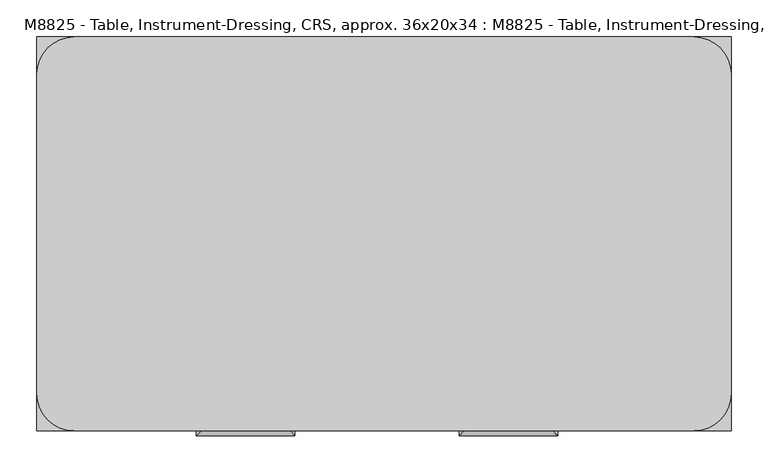
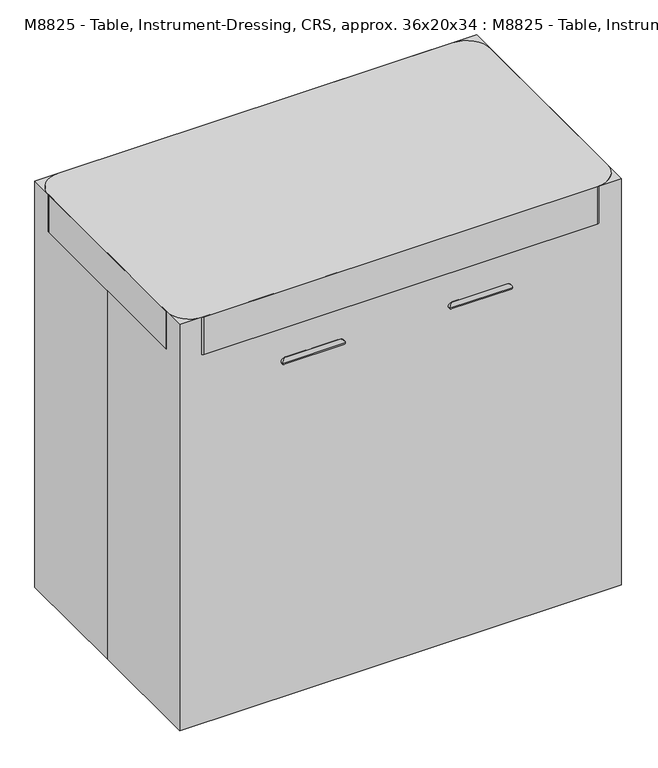
"""IFC4 building model written with IfcOpenShell, lengths in millimetres: proxy geometry, M8825 - Table, Instrument-Dressing, CRS, approx. 36x20x34 : M8825 - Table, Instrument-Dressing, CRS, approx. 36x20x34."""

import ifcopenshell
import ifcopenshell.guid

model = None  # the IFC model being written
_history = None  # IfcOwnerHistory: only IFC2X3 demands one
_inside = {}  # id of a spatial element -> (the spatial element, [elements in it])
_under = {}  # id of a project, library or spatial element -> (it, [spatial elements below it])
_declared = {}  # id of a project -> (the project, [libraries it declares])
_typed = {}  # id of a type object -> (the type object, [elements of that type])
_made_of = {}  # id of a material, layer set ... -> (it, [elements and type objects made of it])


def new_model(schema):
    """Start an empty IFC model of exactly this schema.

    Asked for "IFC4X3", IfcOpenShell would pick the latest addendum, in which some entities
    have other attributes; the version numbers below select the first issue.
    IFC2X3 requires an IfcOwnerHistory on every rooted entity: one is made here for all.
    """
    global model, _history
    if schema == "IFC4X3":
        model = ifcopenshell.file(schema_version=(4, 3, 0, 0))
    else:
        model = ifcopenshell.file(schema=schema)
    _inside.clear()
    _under.clear()
    _declared.clear()
    _typed.clear()
    _made_of.clear()
    _history = None
    if model.schema == "IFC2X3":
        org = make("IfcOrganization", Name="unknown")
        user = make(
            "IfcPersonAndOrganization",
            ThePerson=make("IfcPerson", FamilyName="unknown"),
            TheOrganization=org,
        )
        app = make(
            "IfcApplication",
            ApplicationDeveloper=org,
            Version="unknown",
            ApplicationFullName="unknown",
            ApplicationIdentifier="unknown",
        )
        _history = make(
            "IfcOwnerHistory",
            OwningUser=user,
            OwningApplication=app,
            ChangeAction="ADDED",
            CreationDate=0,
        )
    return model


def make(cls, **values):
    """One entity of the class cls with the attributes given. An attribute that is None is left unset."""
    return model.create_entity(
        cls, **{name: value for name, value in values.items() if value is not None}
    )


def rooted(cls, **values):
    """An entity with a GlobalId (a new one), such as an element, a storey or a relation."""
    return make(cls, GlobalId=ifcopenshell.guid.new(), OwnerHistory=_history, **values)


def si_unit(unit_type, name, prefix=None):
    """IfcSIUnit, for example si_unit("LENGTHUNIT", "METRE", prefix="MILLI")."""
    return make("IfcSIUnit", UnitType=unit_type, Prefix=prefix, Name=name)


def assignment(units):
    """IfcUnitAssignment: the units of a project."""
    return None if units is None else make("IfcUnitAssignment", Units=units)


def point(xyz):
    """IfcCartesianPoint."""
    return None if xyz is None else make("IfcCartesianPoint", Coordinates=xyz)


def direction(xyz):
    """IfcDirection."""
    return None if xyz is None else make("IfcDirection", DirectionRatios=xyz)


def frame(location, z_axis=None, x_axis=None):
    """IfcAxis2Placement3D, a coordinate frame: its origin and axes. An axis left out is left unset."""
    return make(
        "IfcAxis2Placement3D",
        Location=point(location),
        Axis=direction(z_axis),
        RefDirection=direction(x_axis),
    )


def frame_2d(location, x_axis=None):
    """IfcAxis2Placement2D, a coordinate frame in the plane: its origin and x axis."""
    return make(
        "IfcAxis2Placement2D", Location=point(location), RefDirection=direction(x_axis)
    )


def origin():
    """The frame at (0, 0, 0) with its axes left unset."""
    return frame((0.0, 0.0, 0.0))


def origin_with_axes():
    """The frame at (0, 0, 0) with the z axis (0, 0, 1) and the x axis (1, 0, 0) written out."""
    return frame((0.0, 0.0, 0.0), z_axis=(0.0, 0.0, 1.0), x_axis=(1.0, 0.0, 0.0))


def place(relative_to, where):
    """IfcLocalPlacement: puts the frame where relative to a parent placement (None: the world)."""
    return make(
        "IfcLocalPlacement", PlacementRelTo=relative_to, RelativePlacement=where
    )


def context(
    kind, dimensions, precision=None, world=None, true_north=None, identifier=None
):
    """IfcGeometricRepresentationContext, for example the 3D "Model" context."""
    return make(
        "IfcGeometricRepresentationContext",
        ContextIdentifier=identifier,
        ContextType=kind,
        CoordinateSpaceDimension=dimensions,
        Precision=precision,
        WorldCoordinateSystem=world,
        TrueNorth=true_north,
    )


def project(units=None, contexts=None):
    """IfcProject with its units and contexts."""
    return rooted(
        "IfcProject",
        Name="project",
        RepresentationContexts=contexts,
        UnitsInContext=assignment(units),
    )


def spatial(cls, under=None, at=None, **own):
    """A site, building, storey or space (cls), placed at a placement, below another one or the project."""
    s = rooted(cls, ObjectPlacement=at, **own)
    if under is not None:
        _under.setdefault(under.id(), (under, []))[1].append(s)
    return s


def polyline(points):
    """IfcPolyline through the points."""
    return make("IfcPolyline", Points=[point(p) for p in points])


def circle_curve(where, radius):
    """IfcCircle in the frame where."""
    return make("IfcCircle", Position=where, Radius=radius)


def ellipse_curve(where, semi_axis1, semi_axis2):
    """IfcEllipse in the frame where."""
    return make(
        "IfcEllipse", Position=where, SemiAxis1=semi_axis1, SemiAxis2=semi_axis2
    )


def trimmed(basis, trim1, trim2, sense, master):
    """IfcTrimmedCurve: the piece of a basis curve between two trims."""
    return make(
        "IfcTrimmedCurve",
        BasisCurve=basis,
        Trim1=trim1,
        Trim2=trim2,
        SenseAgreement=sense,
        MasterRepresentation=master,
    )


def segment(curve, same_sense, transition):
    """IfcCompositeCurveSegment."""
    return make(
        "IfcCompositeCurveSegment",
        Transition=transition,
        SameSense=same_sense,
        ParentCurve=curve,
    )


def composite_curve(segments, self_intersect=None):
    """IfcCompositeCurve: segments joined end to end."""
    return make("IfcCompositeCurve", Segments=segments, SelfIntersect=self_intersect)


def outline(outer, holes=None, kind="AREA"):
    """IfcArbitraryClosedProfileDef: a profile drawn as a closed curve; with holes, ...WithVoids."""
    if holes is None:
        return make("IfcArbitraryClosedProfileDef", ProfileType=kind, OuterCurve=outer)
    return make(
        "IfcArbitraryProfileDefWithVoids",
        ProfileType=kind,
        OuterCurve=outer,
        InnerCurves=holes,
    )


def extrude(swept, where, along, depth):
    """IfcExtrudedAreaSolid: the profile swept, set in the frame where, extruded along a direction by depth."""
    return make(
        "IfcExtrudedAreaSolid",
        SweptArea=swept,
        Position=where,
        ExtrudedDirection=direction(along),
        Depth=depth,
    )


def shape(context_of_items, identifier, shape_type, items):
    """IfcShapeRepresentation: the items that make up one representation, for example the "Body"."""
    return make(
        "IfcShapeRepresentation",
        ContextOfItems=context_of_items,
        RepresentationIdentifier=identifier,
        RepresentationType=shape_type,
        Items=items,
    )


def source(mapping_origin, context_of_items, identifier, shape_type, items):
    """IfcRepresentationMap: a shape defined once, which mapped items show again and again."""
    return make(
        "IfcRepresentationMap",
        MappingOrigin=mapping_origin,
        MappedRepresentation=shape(context_of_items, identifier, shape_type, items),
    )


def transform(
    local_origin,
    x_axis=None,
    y_axis=None,
    z_axis=None,
    scale=None,
    scale2=None,
    scale3=None,
    uniform=True,
):
    """IfcCartesianTransformationOperator3D, or its non-uniform kind. x_axis, y_axis, z_axis: its Axis1, 2, 3."""
    if uniform:
        return make(
            "IfcCartesianTransformationOperator3D",
            Axis1=direction(x_axis),
            Axis2=direction(y_axis),
            LocalOrigin=point(local_origin),
            Scale=scale,
            Axis3=direction(z_axis),
        )
    return make(
        "IfcCartesianTransformationOperator3DnonUniform",
        Axis1=direction(x_axis),
        Axis2=direction(y_axis),
        LocalOrigin=point(local_origin),
        Scale=scale,
        Axis3=direction(z_axis),
        Scale2=scale2,
        Scale3=scale3,
    )


def mapped(mapping_source, mapping_target):
    """IfcMappedItem: shows the shape of a source again, moved by a transform."""
    return make(
        "IfcMappedItem", MappingSource=mapping_source, MappingTarget=mapping_target
    )


def made_of(thing, what):
    """Note that an element or type object is made of a material, layer set ...; save() writes the relation."""
    if what is not None:
        _made_of.setdefault(what.id(), (what, []))[1].append(thing)
    return thing


def element(
    cls,
    number,
    at=None,
    inside=None,
    cuts=None,
    type_object=None,
    material=None,
    context=None,
    identifier="Body",
    shape_type=None,
    held_by="IfcProductDefinitionShape",
    body=None,
    shapes=None,
    **own,
):
    """One element of the class cls, such as IfcWall. Its Tag is "e" and its number.

    at: its placement. inside: the storey or other place that contains it. cuts: it is an
    opening in that element (IfcRelVoidsElement). A single representation is given by context,
    identifier, shape_type and body (its items); several are given by shapes. held_by: the class
    of the entity that holds the representations. save() writes the other relations.
    """
    e = rooted(cls, Tag="e%d" % number, ObjectPlacement=at, **own)
    if body is not None:
        shapes = [shape(context, identifier, shape_type, body)]
    if shapes is not None:
        e.Representation = make(held_by, Representations=shapes)
    if inside is not None:
        _inside.setdefault(inside.id(), (inside, []))[1].append(e)
    if cuts is not None:
        rooted(
            "IfcRelVoidsElement", RelatingBuildingElement=cuts, RelatedOpeningElement=e
        )
    if type_object is not None:
        _typed.setdefault(type_object.id(), (type_object, []))[1].append(e)
    return made_of(e, material)


def aggregate(whole, parts):
    """IfcRelAggregates: a whole, such as a stair, and the parts it consists of."""
    return rooted("IfcRelAggregates", RelatingObject=whole, RelatedObjects=parts)


def save(model, path):
    """Write the relations noted so far, then the file.

    IfcRelAggregates (storeys below a building ...), IfcRelContainedInSpatialStructure (elements
    in a storey), IfcRelDefinesByType, IfcRelAssociatesMaterial and IfcRelDeclares: one each for
    every whole, place, type object, material and project.
    """
    for whole, parts in _under.values():
        aggregate(whole, parts)
    for where, things in _inside.values():
        rooted(
            "IfcRelContainedInSpatialStructure",
            RelatedElements=things,
            RelatingStructure=where,
        )
    for kind, things in _typed.values():
        rooted("IfcRelDefinesByType", RelatedObjects=things, RelatingType=kind)
    for what, things in _made_of.values():
        rooted("IfcRelAssociatesMaterial", RelatedObjects=things, RelatingMaterial=what)
    for by, libraries in _declared.values():
        rooted("IfcRelDeclares", RelatingContext=by, RelatedDefinitions=libraries)
    model.write(path)


def plane_surface(at):
    """IfcPlane: the flat surface through the origin of the frame at, square to its z axis."""
    return make("IfcPlane", Position=at)


def cylinder_surface(at, radius):
    """IfcCylindricalSurface: all points at the distance radius from the z axis of the frame at."""
    return make("IfcCylindricalSurface", Position=at, Radius=radius)


def advanced_brep(points, edges, surfaces, faces):
    """IfcAdvancedBrep: a solid bounded by faces that lie on surfaces and meet in shared edges.

    An edge is (start, end): straight between two places in points (the first is 0);
    or (start, end, curve); or (start, end, curve, False) where it runs against its curve.
    A face is (place in surfaces, loops), or (place, loops, False) where it looks against
    its surface's normal. A loop lists edges by number (the first is 1), with a minus sign
    where the edge is run from its end to its start. The first loop is the outer one.
    """
    corners = [point(p) for p in points]
    vertices = [make("IfcVertexPoint", VertexGeometry=c) for c in corners]
    made = []
    for start, end, *more in edges:
        made.append(
            make(
                "IfcEdgeCurve",
                EdgeStart=vertices[start],
                EdgeEnd=vertices[end],
                EdgeGeometry=more[0] if more else make("IfcPolyline", Points=[corners[start], corners[end]]),
                SameSense=more[1] if len(more) > 1 else True,
            )
        )
    hull = []
    for where, loops, *sense in faces:
        bounds = []
        for j, loop in enumerate(loops):
            ring = [make("IfcOrientedEdge", EdgeElement=made[abs(k) - 1], Orientation=k > 0) for k in loop]
            bounds.append(
                make(
                    "IfcFaceOuterBound" if j == 0 else "IfcFaceBound",
                    Bound=make("IfcEdgeLoop", EdgeList=ring),
                    Orientation=True,
                )
            )
        hull.append(make("IfcAdvancedFace", Bounds=bounds, FaceSurface=surfaces[where], SameSense=sense[0] if sense else True))
    return make("IfcAdvancedBrep", Outer=make("IfcClosedShell", CfsFaces=hull))


def m8825_table_instrument_dressing_crs_approx_36x20x34_m8825_21174694(model_context):
    return source(origin(), model_context, "Body", "SolidModel", [
        extrude(outline(polyline([(-349.25, 174.4117179), (-349.25, 212.5117179), (349.25, 212.5117179), (349.25, 174.4117179), (400.05, 174.4117179), (400.05, -171.4283546), (349.25, -171.4283546), (349.25, -209.5283546), (-349.25, -209.5283546), (-349.25, -171.4283546), (-400.05, -171.4283546), (-400.05, 174.4117179), (-349.25, 174.4117179)])), frame((0.0, 0.0, 292.1), z_axis=(0.0, 0.0, 1.0), x_axis=(1.0, 0.0, 0.0)), (0.0, 0.0, 1.0), 38.1),
        advanced_brep(
        [(101.6, -228.5783546, 755.65), (114.3, -228.5783546, 755.65), (101.6, -273.05, 755.65), (114.3, -260.35, 755.65), (234.95, -273.05, 755.65), (222.25, -260.35, 755.65), (234.95, -228.5783546, 755.65), (222.25, -228.5783546, 755.65)],
        [
            (0, 1, circle_curve(frame((107.95, -228.5783546, 755.65), z_axis=(0.0, 1.0, 0.0), x_axis=(1.0, 0.0, 0.0)), 6.35)),
            (1, 0, circle_curve(frame((107.95, -228.5783546, 755.65), z_axis=(0.0, 1.0, 0.0), x_axis=(1.0, 0.0, 0.0)), 6.35)),
            (0, 2),
            (2, 3, ellipse_curve(frame((107.95, -266.7, 755.65), z_axis=(-0.7071067811865457, 0.7071067811865492, 0.0), x_axis=(0.7071067811865491, 0.7071067811865458, 0.0)), 8.9802561, 6.35)),
            (3, 1),
            (3, 2, ellipse_curve(frame((107.95, -266.7, 755.65), z_axis=(-0.7071067811865457, 0.7071067811865492, 0.0), x_axis=(0.7071067811865491, 0.7071067811865458, 0.0)), 8.9802561, 6.35)),
            (2, 4),
            (4, 5, ellipse_curve(frame((228.6, -266.7, 755.65), z_axis=(-0.7071067811865492, -0.7071067811865457, 0.0), x_axis=(-0.7071067811865458, 0.7071067811865492, 0.0)), 8.9802561, 6.35)),
            (5, 3),
            (5, 4, ellipse_curve(frame((228.6, -266.7, 755.65), z_axis=(-0.7071067811865492, -0.7071067811865457, 0.0), x_axis=(-0.7071067811865458, 0.7071067811865492, 0.0)), 8.9802561, 6.35)),
            (6, 7, circle_curve(frame((228.6, -228.5783546, 755.65), z_axis=(0.0, 1.0, 0.0), x_axis=(-1.0, 0.0, 0.0)), 6.35)),
            (7, 6, circle_curve(frame((228.6, -228.5783546, 755.65), z_axis=(0.0, 1.0, 0.0), x_axis=(-1.0, 0.0, 0.0)), 6.35)),
            (4, 6),
            (7, 5),
        ],
        [
            plane_surface(frame((107.95, -228.5783546, 755.65), z_axis=(0.0, 1.0, 0.0), x_axis=(0.0, 0.0, 1.0))),
            cylinder_surface(frame((107.95, -228.5783546, 755.65), z_axis=(0.0, 1.0, 0.0), x_axis=(1.0, 0.0, 0.0)), 6.35),
            cylinder_surface(frame((107.95, -266.7, 755.65), z_axis=(-1.0, 0.0, 0.0), x_axis=(0.0, 1.0, 0.0)), 6.35),
            plane_surface(frame((228.6, -228.5783546, 755.65), z_axis=(0.0, 1.0, 0.0), x_axis=(0.0, 0.0, 1.0))),
            cylinder_surface(frame((228.6, -266.7, 755.65), z_axis=(0.0, -1.0, 0.0), x_axis=(-1.0, 0.0, 0.0)), 6.35),
        ],
        [
            (0, [[1, 2]]),
            (1, [[-1, 3, 4, 5]]),
            (1, [[-2, -5, 6, -3]]),
            (2, [[-4, 7, 8, 9]]),
            (2, [[-6, -9, 10, -7]]),
            (3, [[11, 12]]),
            (4, [[-8, 13, -12, 14]]),
            (4, [[-10, -14, -11, -13]]),
        ],
    ),
        extrude(outline(polyline([(328.7951144, -228.5783546), (23.9951144, -228.5783546), (23.9951144, -209.5283546), (328.7951144, -209.5283546), (328.7951144, -228.5783546)])), frame((0.0, 0.0, 714.264534), z_axis=(0.0, 0.0, 1.0), x_axis=(1.0, 0.0, 0.0)), (0.0, 0.0, 1.0), 88.9),
        advanced_brep(
        [(-254.0, -228.5783546, 755.65), (-241.3, -228.5783546, 755.65), (-254.0, -273.05, 755.65), (-241.3, -260.35, 755.65), (-120.65, -273.05, 755.65), (-133.35, -260.35, 755.65), (-120.65, -228.5783546, 755.65), (-133.35, -228.5783546, 755.65)],
        [
            (0, 1, circle_curve(frame((-247.65, -228.5783546, 755.65), z_axis=(0.0, 1.0, 0.0), x_axis=(1.0, 0.0, 0.0)), 6.35)),
            (1, 0, circle_curve(frame((-247.65, -228.5783546, 755.65), z_axis=(0.0, 1.0, 0.0), x_axis=(1.0, 0.0, 0.0)), 6.35)),
            (0, 2),
            (2, 3, ellipse_curve(frame((-247.65, -266.7, 755.65), z_axis=(-0.7071067811865457, 0.7071067811865492, 0.0), x_axis=(0.7071067811865491, 0.7071067811865458, 0.0)), 8.9802561, 6.35)),
            (3, 1),
            (3, 2, ellipse_curve(frame((-247.65, -266.7, 755.65), z_axis=(-0.7071067811865457, 0.7071067811865492, 0.0), x_axis=(0.7071067811865491, 0.7071067811865458, 0.0)), 8.9802561, 6.35)),
            (2, 4),
            (4, 5, ellipse_curve(frame((-127.0, -266.7, 755.65), z_axis=(-0.7071067811865492, -0.7071067811865457, 0.0), x_axis=(-0.7071067811865458, 0.7071067811865492, 0.0)), 8.9802561, 6.35)),
            (5, 3),
            (5, 4, ellipse_curve(frame((-127.0, -266.7, 755.65), z_axis=(-0.7071067811865492, -0.7071067811865457, 0.0), x_axis=(-0.7071067811865458, 0.7071067811865492, 0.0)), 8.9802561, 6.35)),
            (6, 7, circle_curve(frame((-127.0, -228.5783546, 755.65), z_axis=(0.0, 1.0, 0.0), x_axis=(-1.0, 0.0, 0.0)), 6.35)),
            (7, 6, circle_curve(frame((-127.0, -228.5783546, 755.65), z_axis=(0.0, 1.0, 0.0), x_axis=(-1.0, 0.0, 0.0)), 6.35)),
            (4, 6),
            (7, 5),
        ],
        [
            plane_surface(frame((-247.65, -228.5783546, 755.65), z_axis=(0.0, 1.0, 0.0), x_axis=(0.0, 0.0, 1.0))),
            cylinder_surface(frame((-247.65, -228.5783546, 755.65), z_axis=(0.0, 1.0, 0.0), x_axis=(1.0, 0.0, 0.0)), 6.35),
            cylinder_surface(frame((-247.65, -266.7, 755.65), z_axis=(-1.0, 0.0, 0.0), x_axis=(0.0, 1.0, 0.0)), 6.35),
            plane_surface(frame((-127.0, -228.5783546, 755.65), z_axis=(0.0, 1.0, 0.0), x_axis=(0.0, 0.0, 1.0))),
            cylinder_surface(frame((-127.0, -266.7, 755.65), z_axis=(0.0, -1.0, 0.0), x_axis=(-1.0, 0.0, 0.0)), 6.35),
        ],
        [
            (0, [[1, 2]]),
            (1, [[-1, 3, 4, 5]]),
            (1, [[-2, -5, 6, -3]]),
            (2, [[-4, 7, 8, 9]]),
            (2, [[-6, -9, 10, -7]]),
            (3, [[11, 12]]),
            (4, [[-8, 13, -12, 14]]),
            (4, [[-10, -14, -11, -13]]),
        ],
    ),
        extrude(outline(polyline([(-26.8048856, -228.5783546), (-331.6048856, -228.5783546), (-331.6048856, -209.5283546), (-26.8048856, -209.5283546), (-26.8048856, -228.5783546)])), frame((0.0, 0.0, 714.264534), z_axis=(0.0, 0.0, 1.0), x_axis=(1.0, 0.0, 0.0)), (0.0, 0.0, 1.0), 88.9),
        extrude(outline(polyline([(349.25, 193.4617179), (-349.25, 193.4617179), (-349.25, 212.5117179), (349.25, 212.5117179), (349.25, 193.4617179)])), frame((0.0, 0.0, 690.1016667), z_axis=(0.0, 0.0, 1.0), x_axis=(1.0, 0.0, 0.0)), (0.0, 0.0, 1.0), 139.7),
        extrude(outline(polyline([(349.25, -209.5283546), (-349.25, -209.5283546), (-349.25, -190.4783546), (349.25, -190.4783546), (349.25, -209.5283546)])), frame((0.0, 0.0, 690.1016667), z_axis=(0.0, 0.0, 1.0), x_axis=(1.0, 0.0, 0.0)), (0.0, 0.0, 1.0), 139.7),
        extrude(outline(polyline([(381.0, -171.4283546), (381.0, 174.4117179), (400.05, 174.4117179), (400.05, -171.4283546), (381.0, -171.4283546)])), frame((0.0, 0.0, 690.1016667), z_axis=(0.0, 0.0, 1.0), x_axis=(1.0, 0.0, 0.0)), (0.0, 0.0, 1.0), 139.7),
        extrude(outline(polyline([(-381.0, 174.4117179), (-381.0, -171.4283546), (-400.05, -171.4283546), (-400.05, 174.4117179), (-381.0, 174.4117179)])), frame((0.0, 0.0, 690.1016667), z_axis=(0.0, 0.0, 1.0), x_axis=(1.0, 0.0, 0.0)), (0.0, 0.0, 1.0), 139.7),
        extrude(outline(polyline([(349.25, -209.5283546), (349.25, -171.4283546), (400.05, -171.4283546), (400.05, -209.5283546), (349.25, -209.5283546)])), frame((0.0, 0.0, 127.0), z_axis=(0.0, 0.0, 1.0), x_axis=(1.0, 0.0, 0.0)), (0.0, 0.0, 1.0), 702.8016667),
        extrude(outline(polyline([(349.25, 212.5117179), (400.05, 212.5117179), (400.05, 174.4117179), (349.25, 174.4117179), (349.25, 212.5117179)])), frame((0.0, 0.0, 127.0), z_axis=(0.0, 0.0, 1.0), x_axis=(1.0, 0.0, 0.0)), (0.0, 0.0, 1.0), 702.8016667),
        extrude(outline(polyline([(-349.25, -209.5283546), (-400.05, -209.5283546), (-400.05, -171.4283546), (-349.25, -171.4283546), (-349.25, -209.5283546)])), frame((0.0, 0.0, 127.0), z_axis=(0.0, 0.0, 1.0), x_axis=(1.0, 0.0, 0.0)), (0.0, 0.0, 1.0), 702.8016667),
        extrude(outline(polyline([(-349.25, 212.5117179), (-349.25, 174.4117179), (-400.05, 174.4117179), (-400.05, 212.5117179), (-349.25, 212.5117179)])), frame((0.0, 0.0, 127.0), z_axis=(0.0, 0.0, 1.0), x_axis=(1.0, 0.0, 0.0)), (0.0, 0.0, 1.0), 702.8016667),
        extrude(outline(composite_curve([segment(trimmed(circle_curve(frame_2d((-366.1833333, 193.6533546)), 16.9333333), [point((-366.1833333, 210.5866879))], [point((-366.1833333, 176.7200213))], False, "CARTESIAN"), True, "CONTINUOUS"), segment(trimmed(circle_curve(frame_2d((-366.1833333, 193.6533546)), 16.9333333), [point((-366.1833333, 176.7200213))], [point((-366.1833333, 210.5866879))], False, "CARTESIAN"), True, "CONTINUOUS")], self_intersect=False)), frame((0.0, 0.0, 84.8149176), z_axis=(0.0, 0.0, 1.0), x_axis=(1.0, 0.0, 0.0)), (0.0, 0.0, 1.0), 42.1850824),
        extrude(outline(composite_curve([segment(trimmed(circle_curve(frame_2d((-366.1833333, -190.4783546)), 16.9333333), [point((-366.1833333, -207.4116879))], [point((-366.1833333, -173.5450213))], False, "CARTESIAN"), True, "CONTINUOUS"), segment(trimmed(circle_curve(frame_2d((-366.1833333, -190.4783546)), 16.9333333), [point((-366.1833333, -173.5450213))], [point((-366.1833333, -207.4116879))], False, "CARTESIAN"), True, "CONTINUOUS")], self_intersect=False)), frame((0.0, 0.0, 84.8149176), z_axis=(0.0, 0.0, 1.0), x_axis=(1.0, 0.0, 0.0)), (0.0, 0.0, 1.0), 42.1850824),
        extrude(outline(composite_curve([segment(trimmed(circle_curve(frame_2d((50.8, -349.25)), 50.8), [point((50.8, -400.05))], [point((50.8, -298.45))], False, "CARTESIAN"), True, "CONTINUOUS"), segment(trimmed(circle_curve(frame_2d((50.8, -349.25)), 50.8), [point((50.8, -298.45))], [point((50.8, -400.05))], False, "CARTESIAN"), True, "CONTINUOUS")], self_intersect=False)), frame((0.0, -171.45, 0.0), z_axis=(0.0, 1.0, 0.0), x_axis=(0.0, 0.0, 1.0)), (0.0, 0.0, 1.0), 19.05),
        extrude(outline(composite_curve([segment(trimmed(circle_curve(frame_2d((50.8, -349.25)), 50.8), [point((50.8, -400.05))], [point((50.8, -298.45))], False, "CARTESIAN"), True, "CONTINUOUS"), segment(trimmed(circle_curve(frame_2d((50.8, -349.25)), 50.8), [point((50.8, -298.45))], [point((50.8, -400.05))], False, "CARTESIAN"), True, "CONTINUOUS")], self_intersect=False)), frame((0.0, -228.6, 0.0), z_axis=(0.0, 1.0, 0.0), x_axis=(0.0, 0.0, 1.0)), (0.0, 0.0, 1.0), 19.05),
        extrude(outline(composite_curve([segment(trimmed(circle_curve(frame_2d((50.8, -349.25)), 33.8666667), [point((50.8, -315.3833333))], [point((50.8, -383.1166667))], False, "CARTESIAN"), True, "CONTINUOUS"), segment(trimmed(circle_curve(frame_2d((50.8, -349.25)), 33.8666667), [point((50.8, -383.1166667))], [point((50.8, -315.3833333))], False, "CARTESIAN"), True, "CONTINUOUS")], self_intersect=False)), frame((0.0, -209.55, 0.0), z_axis=(0.0, 1.0, 0.0), x_axis=(0.0, 0.0, 1.0)), (0.0, 0.0, 1.0), 38.1),
        extrude(outline(composite_curve([segment(trimmed(circle_curve(frame_2d((50.8, -349.25)), 50.8), [point((50.8, -400.05))], [point((50.8, -298.45))], False, "CARTESIAN"), True, "CONTINUOUS"), segment(trimmed(circle_curve(frame_2d((50.8, -349.25)), 50.8), [point((50.8, -298.45))], [point((50.8, -400.05))], False, "CARTESIAN"), True, "CONTINUOUS")], self_intersect=False)), frame((0.0, 155.3617179, 0.0), z_axis=(0.0, 1.0, 0.0), x_axis=(0.0, 0.0, 1.0)), (0.0, 0.0, 1.0), 19.05),
        extrude(outline(composite_curve([segment(trimmed(circle_curve(frame_2d((50.8, -349.25)), 50.8), [point((50.8, -400.05))], [point((50.8, -298.45))], False, "CARTESIAN"), True, "CONTINUOUS"), segment(trimmed(circle_curve(frame_2d((50.8, -349.25)), 50.8), [point((50.8, -298.45))], [point((50.8, -400.05))], False, "CARTESIAN"), True, "CONTINUOUS")], self_intersect=False)), frame((0.0, 212.5117179, 0.0), z_axis=(0.0, 1.0, 0.0), x_axis=(0.0, 0.0, 1.0)), (0.0, 0.0, 1.0), 19.05),
        extrude(outline(composite_curve([segment(trimmed(circle_curve(frame_2d((50.8, -349.25)), 33.8666667), [point((50.8, -315.3833333))], [point((50.8, -383.1166667))], False, "CARTESIAN"), True, "CONTINUOUS"), segment(trimmed(circle_curve(frame_2d((50.8, -349.25)), 33.8666667), [point((50.8, -383.1166667))], [point((50.8, -315.3833333))], False, "CARTESIAN"), True, "CONTINUOUS")], self_intersect=False)), frame((0.0, 174.4117179, 0.0), z_axis=(0.0, 1.0, 0.0), x_axis=(0.0, 0.0, 1.0)), (0.0, 0.0, 1.0), 38.1),
        extrude(outline(composite_curve([segment(trimmed(circle_curve(frame_2d((366.1833333, 193.6533546)), 16.9333333), [point((366.1833333, 210.5866879))], [point((366.1833333, 176.7200213))], False, "CARTESIAN"), True, "CONTINUOUS"), segment(trimmed(circle_curve(frame_2d((366.1833333, 193.6533546)), 16.9333333), [point((366.1833333, 176.7200213))], [point((366.1833333, 210.5866879))], False, "CARTESIAN"), True, "CONTINUOUS")], self_intersect=False)), frame((0.0, 0.0, 84.8149176), z_axis=(0.0, 0.0, 1.0), x_axis=(1.0, 0.0, 0.0)), (0.0, 0.0, 1.0), 42.1850824),
        extrude(outline(composite_curve([segment(trimmed(circle_curve(frame_2d((366.1833333, -190.4783546)), 16.9333333), [point((366.1833333, -207.4116879))], [point((366.1833333, -173.5450213))], False, "CARTESIAN"), True, "CONTINUOUS"), segment(trimmed(circle_curve(frame_2d((366.1833333, -190.4783546)), 16.9333333), [point((366.1833333, -173.5450213))], [point((366.1833333, -207.4116879))], False, "CARTESIAN"), True, "CONTINUOUS")], self_intersect=False)), frame((0.0, 0.0, 84.8149176), z_axis=(0.0, 0.0, 1.0), x_axis=(1.0, 0.0, 0.0)), (0.0, 0.0, 1.0), 42.1850824),
        extrude(outline(composite_curve([segment(trimmed(circle_curve(frame_2d((50.8, 349.25)), 50.8), [point((50.8, 400.05))], [point((50.8, 298.45))], False, "CARTESIAN"), True, "CONTINUOUS"), segment(trimmed(circle_curve(frame_2d((50.8, 349.25)), 50.8), [point((50.8, 298.45))], [point((50.8, 400.05))], False, "CARTESIAN"), True, "CONTINUOUS")], self_intersect=False)), frame((0.0, -171.45, 0.0), z_axis=(0.0, 1.0, 0.0), x_axis=(0.0, 0.0, 1.0)), (0.0, 0.0, 1.0), 19.05),
        extrude(outline(composite_curve([segment(trimmed(circle_curve(frame_2d((50.8, 349.25)), 50.8), [point((50.8, 400.05))], [point((50.8, 298.45))], False, "CARTESIAN"), True, "CONTINUOUS"), segment(trimmed(circle_curve(frame_2d((50.8, 349.25)), 50.8), [point((50.8, 298.45))], [point((50.8, 400.05))], False, "CARTESIAN"), True, "CONTINUOUS")], self_intersect=False)), frame((0.0, -228.6, 0.0), z_axis=(0.0, 1.0, 0.0), x_axis=(0.0, 0.0, 1.0)), (0.0, 0.0, 1.0), 19.05),
        extrude(outline(composite_curve([segment(trimmed(circle_curve(frame_2d((50.8, 349.25)), 33.8666667), [point((50.8, 315.3833333))], [point((50.8, 383.1166667))], False, "CARTESIAN"), True, "CONTINUOUS"), segment(trimmed(circle_curve(frame_2d((50.8, 349.25)), 33.8666667), [point((50.8, 383.1166667))], [point((50.8, 315.3833333))], False, "CARTESIAN"), True, "CONTINUOUS")], self_intersect=False)), frame((0.0, -209.55, 0.0), z_axis=(0.0, 1.0, 0.0), x_axis=(0.0, 0.0, 1.0)), (0.0, 0.0, 1.0), 38.1),
        extrude(outline(composite_curve([segment(trimmed(circle_curve(frame_2d((50.8, 349.25)), 50.8), [point((50.8, 400.05))], [point((50.8, 298.45))], False, "CARTESIAN"), True, "CONTINUOUS"), segment(trimmed(circle_curve(frame_2d((50.8, 349.25)), 50.8), [point((50.8, 298.45))], [point((50.8, 400.05))], False, "CARTESIAN"), True, "CONTINUOUS")], self_intersect=False)), frame((0.0, 155.3617179, 0.0), z_axis=(0.0, 1.0, 0.0), x_axis=(0.0, 0.0, 1.0)), (0.0, 0.0, 1.0), 19.05),
        extrude(outline(composite_curve([segment(trimmed(circle_curve(frame_2d((50.8, 349.25)), 50.8), [point((50.8, 400.05))], [point((50.8, 298.45))], False, "CARTESIAN"), True, "CONTINUOUS"), segment(trimmed(circle_curve(frame_2d((50.8, 349.25)), 50.8), [point((50.8, 298.45))], [point((50.8, 400.05))], False, "CARTESIAN"), True, "CONTINUOUS")], self_intersect=False)), frame((0.0, 212.5117179, 0.0), z_axis=(0.0, 1.0, 0.0), x_axis=(0.0, 0.0, 1.0)), (0.0, 0.0, 1.0), 19.05),
        extrude(outline(composite_curve([segment(trimmed(circle_curve(frame_2d((50.8, 349.25)), 33.8666667), [point((50.8, 315.3833333))], [point((50.8, 383.1166667))], False, "CARTESIAN"), True, "CONTINUOUS"), segment(trimmed(circle_curve(frame_2d((50.8, 349.25)), 33.8666667), [point((50.8, 383.1166667))], [point((50.8, 315.3833333))], False, "CARTESIAN"), True, "CONTINUOUS")], self_intersect=False)), frame((0.0, 174.4117179, 0.0), z_axis=(0.0, 1.0, 0.0), x_axis=(0.0, 0.0, 1.0)), (0.0, 0.0, 1.0), 38.1),
        extrude(outline(composite_curve([segment(trimmed(circle_curve(frame_2d((419.1, 215.9)), 50.8), [point((419.1, 266.7))], [point((469.9, 215.9))], False, "CARTESIAN"), True, "CONTINUOUS"), segment(polyline([(469.9, 215.9), (469.9, -215.9)]), True, "CONTINUOUS"), segment(trimmed(circle_curve(frame_2d((419.1, -215.9)), 50.8), [point((469.9, -215.9))], [point((419.1, -266.7))], False, "CARTESIAN"), True, "CONTINUOUS"), segment(polyline([(419.1, -266.7), (-419.1, -266.7)]), True, "CONTINUOUS"), segment(trimmed(circle_curve(frame_2d((-419.1, -215.9)), 50.8), [point((-419.1, -266.7))], [point((-469.9, -215.9))], False, "CARTESIAN"), True, "CONTINUOUS"), segment(polyline([(-469.9, -215.9), (-469.9, 215.9)]), True, "CONTINUOUS"), segment(trimmed(circle_curve(frame_2d((-419.1, 215.9)), 50.8), [point((-469.9, 215.9))], [point((-419.1, 266.7))], False, "CARTESIAN"), True, "CONTINUOUS"), segment(polyline([(-419.1, 266.7), (419.1, 266.7)]), True, "CONTINUOUS")], self_intersect=False)), frame((0.0, 0.0, 829.8016667), z_axis=(0.0, 0.0, 1.0), x_axis=(1.0, 0.0, 0.0)), (0.0, 0.0, 1.0), 84.5983333),
        extrude(outline(polyline([(-469.9, 266.7), (469.9, 266.7), (469.9, -266.7), (-469.9, -266.7), (-469.9, 0.0), (-469.9, 266.7)])), origin_with_axes(), (0.0, 0.0, 1.0), 914.4),
    ])


if __name__ == "__main__":
    model = new_model("IFC4")
    model_context = context("Model", 3, world=origin())
    ifc_project = project(units=[si_unit("LENGTHUNIT", "METRE", prefix="MILLI")], contexts=[model_context])
    site = spatial("IfcSite", under=ifc_project)
    building = spatial("IfcBuilding", under=site)
    placement = place(None, origin())
    m8825_table_instrument_dressing_crs_approx_36x20x34_m8825_shape = m8825_table_instrument_dressing_crs_approx_36x20x34_m8825_21174694(model_context)
    element("IfcBuildingElementProxy", 1, Name="M8825 - Table, Instrument-Dressing, CRS, approx. 36x20x34 : M8825 - Table, Instrument-Dressing, CRS, approx. 36x20x34", ObjectType="M8825 - Table, Instrument-Dressing, CRS, approx. 36x20x34 : M8825 - Table, Instrument-Dressing, CRS, approx. 36x20x34", at=placement, inside=building, context=model_context, shape_type="MappedRepresentation", body=[
        mapped(m8825_table_instrument_dressing_crs_approx_36x20x34_m8825_shape, transform((0.0, 0.0, 0.0), x_axis=(1.0, 0.0, 0.0), y_axis=(0.0, 1.0, 0.0), z_axis=(0.0, 0.0, 1.0))),
    ])
    save(model, "model.ifc")

# Revit data of these elements
# Project information
#   Room Abbreviation = "XDCY1"
#   Room Description = "Xray, Cystology (XDCY1)"
#   Sheets - Total = "6"
#   Project Issue Date = "Issue Date"
#   Project Status = "Project Status"
#   Client Name = "Owner"
#   Project Address = "Enter address here"
#   Project Name = "Project Name"
#   Project Number = "Project Number"
#   Publication Date = "1-Feb-16"
# Type "M8825 - Table, Instrument-Dressing, CRS, approx. 36x20x34 : M8825 - Table, Instrument-Dressing, CRS, approx. 36x20x34"
#   Watts2 = "0"
#   Watts1 = "0"
#   Unit_Issue = "EA"
#   UTIL_6_Misc = "-"
#   UTIL_5_NonMedGas = "-"
#   UTIL_4_MiscGas = "-"
#   UTIL_3_MedGas = "-"
#   UTIL_2_Elec = "-"
#   UTIL_1_WaterDrain = "-"
#   Nomenclature = "Table, Instrument/Dressing, CRS, approx. 36x20x34"
#   NSN = "6530"
#   Location [instance default] = ""
#   JSN = "M8825"
#   Fund_Source_VA = "-"
#   Fund_Source_Navy = "-"
#   Fund_Source_Army = "-"
#   Fund_Source_AF = "-"
#   ELEC_Volts2 = "0"
#   ELEC_Volts1 = "0"
#   ELEC_Phase2 = "0"
#   ELEC_Phase1 = "0"
#   ELEC_HertzSwitch = "0"
#   ELEC_HertzDependent = "0"
#   ELEC_Hertz = "0"
#   ELEC_Amps2 = "0"
#   ELEC_Amps1 = "0"
#   DetailDescription = "Instrument and dressing table. Made of corrosion resistant stainless steel with a sound deadened top. Includes guard rail, shelf and two side-by-side drawers. The table is mounted on swivel, ball-bearing casters."
#   CAT_VA = "C"
#   CAT_Navy = "C"
#   CAT_IHS = "-"
#   CAT_Army = "C"
#   CAT_AF = "C"
#   BTUperhour = "0"
#   radius = 0' - 2"
#   calc 2 = 0' - 0.66667"
#   calc 1 = 0' - 1.33333"
#   Weight_IP = 90
#   DIM_Width_IP = 3' - 1"
#   DIM_Height_IP = 3' - 0"
#   DIM_Depth_IP = 1' - 9"
#   top [instance default] = none
#   finish [instance default] = none
# Element 1 (IfcBuildingElementProxy, "M8825 - Table, Instrument-Dressing, CRS, approx. 36x20x34 : M8825 - Table, Instrument-Dressing, CRS, approx. 36x20x34")
#   Location = "XDCY1"
#   Materials on its faces: "EquipSpace"
# Materials
#   "EquipSpace": class "Unassigned", colour RGB 221 217 195, transparency 0.5
